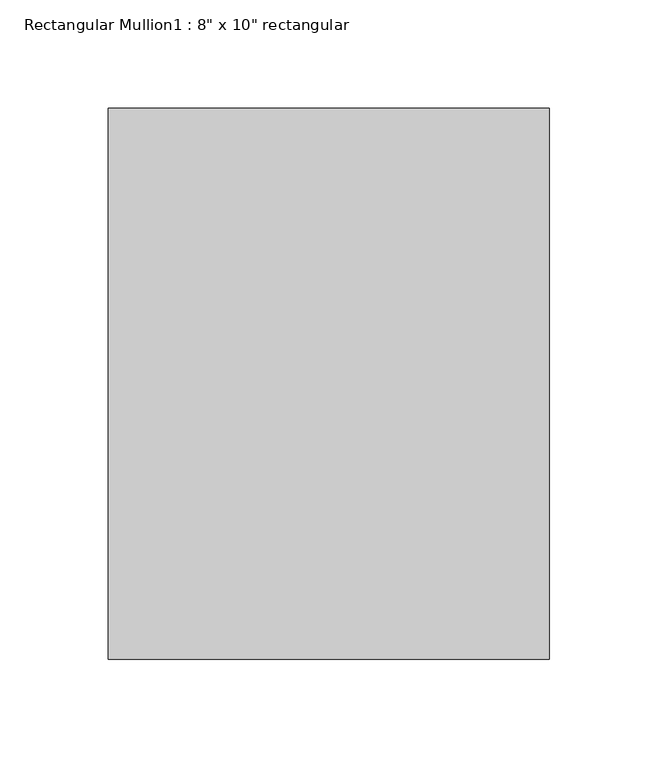
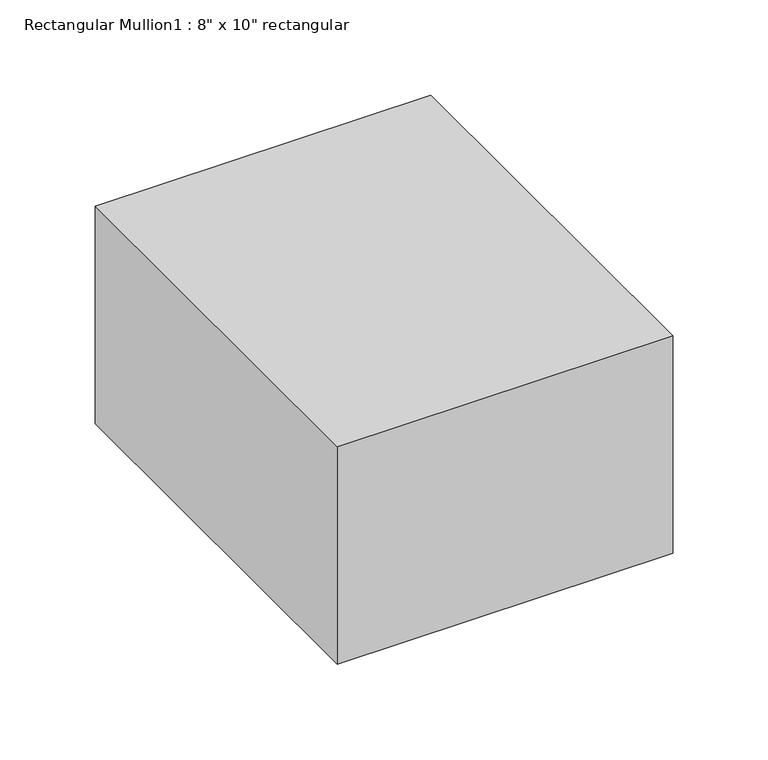
"""IFC4 building model written with IfcOpenShell, lengths in millimetres: member geometry."""

import ifcopenshell
import ifcopenshell.guid

model = None  # the IFC model being written
_history = None  # IfcOwnerHistory: only IFC2X3 demands one
_inside = {}  # id of a spatial element -> (the spatial element, [elements in it])
_under = {}  # id of a project, library or spatial element -> (it, [spatial elements below it])
_declared = {}  # id of a project -> (the project, [libraries it declares])
_typed = {}  # id of a type object -> (the type object, [elements of that type])
_made_of = {}  # id of a material, layer set ... -> (it, [elements and type objects made of it])


def new_model(schema):
    """Start an empty IFC model of exactly this schema.

    Asked for "IFC4X3", IfcOpenShell would pick the latest addendum, in which some entities
    have other attributes; the version numbers below select the first issue.
    IFC2X3 requires an IfcOwnerHistory on every rooted entity: one is made here for all.
    """
    global model, _history
    if schema == "IFC4X3":
        model = ifcopenshell.file(schema_version=(4, 3, 0, 0))
    else:
        model = ifcopenshell.file(schema=schema)
    _inside.clear()
    _under.clear()
    _declared.clear()
    _typed.clear()
    _made_of.clear()
    _history = None
    if model.schema == "IFC2X3":
        org = make("IfcOrganization", Name="unknown")
        user = make(
            "IfcPersonAndOrganization",
            ThePerson=make("IfcPerson", FamilyName="unknown"),
            TheOrganization=org,
        )
        app = make(
            "IfcApplication",
            ApplicationDeveloper=org,
            Version="unknown",
            ApplicationFullName="unknown",
            ApplicationIdentifier="unknown",
        )
        _history = make(
            "IfcOwnerHistory",
            OwningUser=user,
            OwningApplication=app,
            ChangeAction="ADDED",
            CreationDate=0,
        )
    return model


def make(cls, **values):
    """One entity of the class cls with the attributes given. An attribute that is None is left unset."""
    return model.create_entity(
        cls, **{name: value for name, value in values.items() if value is not None}
    )


def rooted(cls, **values):
    """An entity with a GlobalId (a new one), such as an element, a storey or a relation."""
    return make(cls, GlobalId=ifcopenshell.guid.new(), OwnerHistory=_history, **values)


def si_unit(unit_type, name, prefix=None):
    """IfcSIUnit, for example si_unit("LENGTHUNIT", "METRE", prefix="MILLI")."""
    return make("IfcSIUnit", UnitType=unit_type, Prefix=prefix, Name=name)


def assignment(units):
    """IfcUnitAssignment: the units of a project."""
    return None if units is None else make("IfcUnitAssignment", Units=units)


def point(xyz):
    """IfcCartesianPoint."""
    return None if xyz is None else make("IfcCartesianPoint", Coordinates=xyz)


def direction(xyz):
    """IfcDirection."""
    return None if xyz is None else make("IfcDirection", DirectionRatios=xyz)


def frame(location, z_axis=None, x_axis=None):
    """IfcAxis2Placement3D, a coordinate frame: its origin and axes. An axis left out is left unset."""
    return make(
        "IfcAxis2Placement3D",
        Location=point(location),
        Axis=direction(z_axis),
        RefDirection=direction(x_axis),
    )


def origin():
    """The frame at (0, 0, 0) with its axes left unset."""
    return frame((0.0, 0.0, 0.0))


def place(relative_to, where):
    """IfcLocalPlacement: puts the frame where relative to a parent placement (None: the world)."""
    return make(
        "IfcLocalPlacement", PlacementRelTo=relative_to, RelativePlacement=where
    )


def context(
    kind, dimensions, precision=None, world=None, true_north=None, identifier=None
):
    """IfcGeometricRepresentationContext, for example the 3D "Model" context."""
    return make(
        "IfcGeometricRepresentationContext",
        ContextIdentifier=identifier,
        ContextType=kind,
        CoordinateSpaceDimension=dimensions,
        Precision=precision,
        WorldCoordinateSystem=world,
        TrueNorth=true_north,
    )


def project(units=None, contexts=None):
    """IfcProject with its units and contexts."""
    return rooted(
        "IfcProject",
        Name="project",
        RepresentationContexts=contexts,
        UnitsInContext=assignment(units),
    )


def spatial(cls, under=None, at=None, **own):
    """A site, building, storey or space (cls), placed at a placement, below another one or the project."""
    s = rooted(cls, ObjectPlacement=at, **own)
    if under is not None:
        _under.setdefault(under.id(), (under, []))[1].append(s)
    return s


def polyline(points):
    """IfcPolyline through the points."""
    return make("IfcPolyline", Points=[point(p) for p in points])


def outline(outer, holes=None, kind="AREA"):
    """IfcArbitraryClosedProfileDef: a profile drawn as a closed curve; with holes, ...WithVoids."""
    if holes is None:
        return make("IfcArbitraryClosedProfileDef", ProfileType=kind, OuterCurve=outer)
    return make(
        "IfcArbitraryProfileDefWithVoids",
        ProfileType=kind,
        OuterCurve=outer,
        InnerCurves=holes,
    )


def extrude(swept, where, along, depth):
    """IfcExtrudedAreaSolid: the profile swept, set in the frame where, extruded along a direction by depth."""
    return make(
        "IfcExtrudedAreaSolid",
        SweptArea=swept,
        Position=where,
        ExtrudedDirection=direction(along),
        Depth=depth,
    )


def shape(context_of_items, identifier, shape_type, items):
    """IfcShapeRepresentation: the items that make up one representation, for example the "Body"."""
    return make(
        "IfcShapeRepresentation",
        ContextOfItems=context_of_items,
        RepresentationIdentifier=identifier,
        RepresentationType=shape_type,
        Items=items,
    )


def source(mapping_origin, context_of_items, identifier, shape_type, items):
    """IfcRepresentationMap: a shape defined once, which mapped items show again and again."""
    return make(
        "IfcRepresentationMap",
        MappingOrigin=mapping_origin,
        MappedRepresentation=shape(context_of_items, identifier, shape_type, items),
    )


def transform(
    local_origin,
    x_axis=None,
    y_axis=None,
    z_axis=None,
    scale=None,
    scale2=None,
    scale3=None,
    uniform=True,
):
    """IfcCartesianTransformationOperator3D, or its non-uniform kind. x_axis, y_axis, z_axis: its Axis1, 2, 3."""
    if uniform:
        return make(
            "IfcCartesianTransformationOperator3D",
            Axis1=direction(x_axis),
            Axis2=direction(y_axis),
            LocalOrigin=point(local_origin),
            Scale=scale,
            Axis3=direction(z_axis),
        )
    return make(
        "IfcCartesianTransformationOperator3DnonUniform",
        Axis1=direction(x_axis),
        Axis2=direction(y_axis),
        LocalOrigin=point(local_origin),
        Scale=scale,
        Axis3=direction(z_axis),
        Scale2=scale2,
        Scale3=scale3,
    )


def mapped(mapping_source, mapping_target):
    """IfcMappedItem: shows the shape of a source again, moved by a transform."""
    return make(
        "IfcMappedItem", MappingSource=mapping_source, MappingTarget=mapping_target
    )


def made_of(thing, what):
    """Note that an element or type object is made of a material, layer set ...; save() writes the relation."""
    if what is not None:
        _made_of.setdefault(what.id(), (what, []))[1].append(thing)
    return thing


def element(
    cls,
    number,
    at=None,
    inside=None,
    cuts=None,
    type_object=None,
    material=None,
    context=None,
    identifier="Body",
    shape_type=None,
    held_by="IfcProductDefinitionShape",
    body=None,
    shapes=None,
    **own,
):
    """One element of the class cls, such as IfcWall. Its Tag is "e" and its number.

    at: its placement. inside: the storey or other place that contains it. cuts: it is an
    opening in that element (IfcRelVoidsElement). A single representation is given by context,
    identifier, shape_type and body (its items); several are given by shapes. held_by: the class
    of the entity that holds the representations. save() writes the other relations.
    """
    e = rooted(cls, Tag="e%d" % number, ObjectPlacement=at, **own)
    if body is not None:
        shapes = [shape(context, identifier, shape_type, body)]
    if shapes is not None:
        e.Representation = make(held_by, Representations=shapes)
    if inside is not None:
        _inside.setdefault(inside.id(), (inside, []))[1].append(e)
    if cuts is not None:
        rooted(
            "IfcRelVoidsElement", RelatingBuildingElement=cuts, RelatedOpeningElement=e
        )
    if type_object is not None:
        _typed.setdefault(type_object.id(), (type_object, []))[1].append(e)
    return made_of(e, material)


def aggregate(whole, parts):
    """IfcRelAggregates: a whole, such as a stair, and the parts it consists of."""
    return rooted("IfcRelAggregates", RelatingObject=whole, RelatedObjects=parts)


def save(model, path):
    """Write the relations noted so far, then the file.

    IfcRelAggregates (storeys below a building ...), IfcRelContainedInSpatialStructure (elements
    in a storey), IfcRelDefinesByType, IfcRelAssociatesMaterial and IfcRelDeclares: one each for
    every whole, place, type object, material and project.
    """
    for whole, parts in _under.values():
        aggregate(whole, parts)
    for where, things in _inside.values():
        rooted(
            "IfcRelContainedInSpatialStructure",
            RelatedElements=things,
            RelatingStructure=where,
        )
    for kind, things in _typed.values():
        rooted("IfcRelDefinesByType", RelatedObjects=things, RelatingType=kind)
    for what, things in _made_of.values():
        rooted("IfcRelAssociatesMaterial", RelatedObjects=things, RelatingMaterial=what)
    for by, libraries in _declared.values():
        rooted("IfcRelDeclares", RelatingContext=by, RelatedDefinitions=libraries)
    model.write(path)


def member_eb4aacb2(model_context):
    return source(origin(), model_context, "Body", "SweptSolid", [
        extrude(outline(polyline([(101.6, 127.0), (101.6, -127.0), (-101.6, -127.0), (-101.6, 127.0), (101.6, 127.0)])), frame((0.0, 0.0, -139.2998379), z_axis=(0.0, 0.0, 1.0), x_axis=(1.0, 0.0, 0.0)), (0.0, 0.0, 1.0), 139.2998379),
    ])


if __name__ == "__main__":
    model = new_model("IFC4")
    model_context = context("Model", 3, world=origin())
    ifc_project = project(units=[si_unit("LENGTHUNIT", "METRE", prefix="MILLI")], contexts=[model_context])
    site = spatial("IfcSite", under=ifc_project)
    building = spatial("IfcBuilding", under=site)
    placement = place(None, origin())
    member_shape = member_eb4aacb2(model_context)
    element("IfcMember", 1, ObjectType="Rectangular Mullion1 : 8\" x 10\" rectangular", at=placement, inside=building, context=model_context, shape_type="MappedRepresentation", body=[
        mapped(member_shape, transform((0.0, 0.0, 0.0), x_axis=(1.0, 0.0, 0.0), y_axis=(0.0, 1.0, 0.0), z_axis=(0.0, 0.0, 1.0))),
    ])
    save(model, "model.ifc")

# Revit data of these elements
# Type "Rectangular Mullion1 : 8\" x 10\" rectangular"
#   built-in parameter 1007304 = 0.833333 (stored number, unit not read)
#   built-in parameter 1007301 = 0.333333 (stored number, unit not read)
#   built-in parameter 1007300 = 0.333333 (stored number, unit not read)
# Element 1 (IfcMember, "Rectangular Mullion1 : 8\" x 10\" rectangular")
#   Materials on its faces: "support-frame"
# Materials
#   "support-frame": class "Unassigned", colour RGB 233 233 233, transparency 0, Cost = 0
